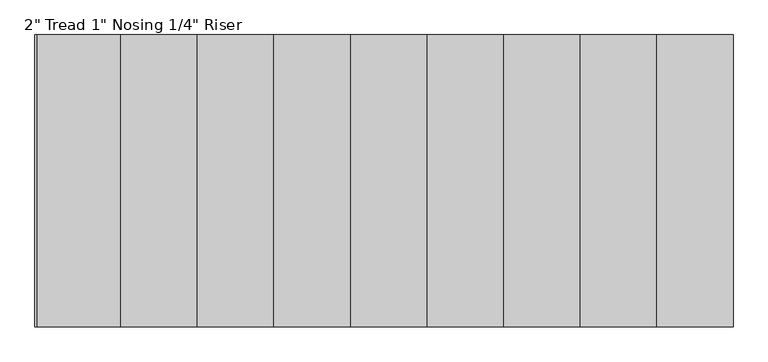
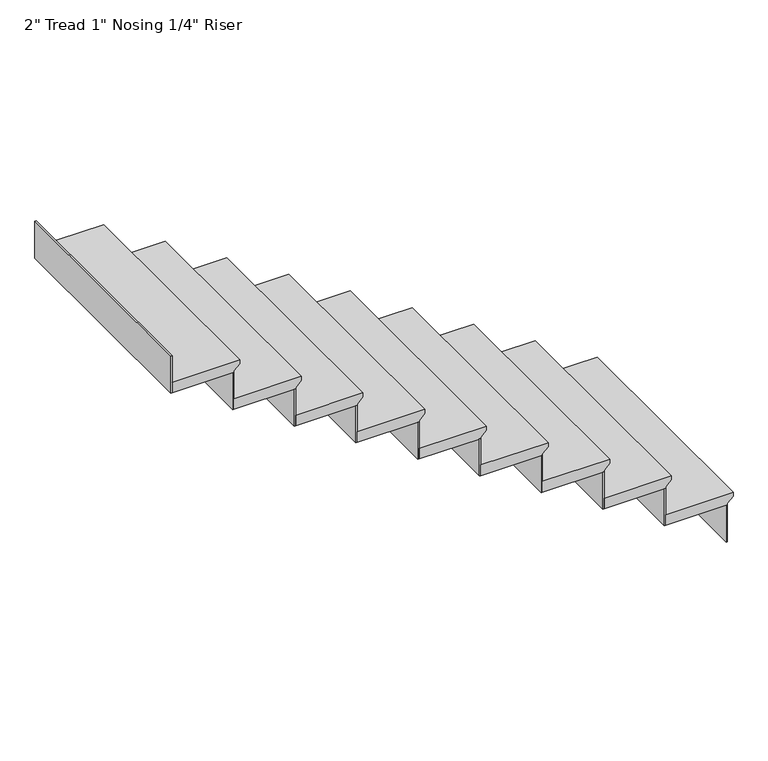
"""IFC4 building model written with IfcOpenShell, lengths in millimetres: stair flight geometry."""

from ifc_helpers import new_model, si_unit, frame, origin, place, context, project, spatial, polyline, outline, extrude, source, transform, mapped, element, save


def stair_flight_a874c81b(model_context):
    return source(origin(), model_context, "Body", "SweptSolid", [
        extrude(outline(polyline([(4959.1783784, 665956.388677), (4959.1783784, 665651.588677), (4908.3783784, 665651.588677), (4908.3783784, 665930.988677), (4914.7283784, 665930.988677), (4940.1283784, 665956.388677), (4959.1783784, 665956.388677)])), frame((0.0, -550482.8413841, 0.0), z_axis=(0.0, 1.0, 0.0), x_axis=(0.0, 0.0, 1.0)), (0.0, 0.0, 1.0), 1066.8),
        extrude(outline(polyline([(665924.638677, -549416.0413841), (665930.988677, -549416.0413841), (665930.988677, -550482.8413841), (665924.638677, -550482.8413841), (665924.638677, -549416.0413841)])), frame((0.0, 0.0, 4731.2648649), z_axis=(0.0, 0.0, 1.0), x_axis=(1.0, 0.0, 0.0)), (0.0, 0.0, 1.0), 177.1135135),
        extrude(outline(polyline([(665645.238677, -549416.0413841), (665651.588677, -549416.0413841), (665651.588677, -550482.8413841), (665645.238677, -550482.8413841), (665645.238677, -549416.0413841)])), frame((0.0, 0.0, 4908.3783784), z_axis=(0.0, 0.0, 1.0), x_axis=(1.0, 0.0, 0.0)), (0.0, 0.0, 1.0), 177.1135135),
        extrude(outline(polyline([(5136.2918919, 665676.988677), (5136.2918919, 665372.188677), (5085.4918919, 665372.188677), (5085.4918919, 665651.588677), (5091.8418919, 665651.588677), (5117.2418919, 665676.988677), (5136.2918919, 665676.988677)])), frame((0.0, -550482.8413841, 0.0), z_axis=(0.0, 1.0, 0.0), x_axis=(0.0, 0.0, 1.0)), (0.0, 0.0, 1.0), 1066.8),
        extrude(outline(polyline([(665365.838677, -549416.0413841), (665372.188677, -549416.0413841), (665372.188677, -550482.8413841), (665365.838677, -550482.8413841), (665365.838677, -549416.0413841)])), frame((0.0, 0.0, 5085.4918919), z_axis=(0.0, 0.0, 1.0), x_axis=(1.0, 0.0, 0.0)), (0.0, 0.0, 1.0), 177.1135135),
        extrude(outline(polyline([(5313.4054054, 665397.588677), (5313.4054054, 665092.788677), (5262.6054054, 665092.788677), (5262.6054054, 665372.188677), (5268.9554054, 665372.188677), (5294.3554054, 665397.588677), (5313.4054054, 665397.588677)])), frame((0.0, -550482.8413841, 0.0), z_axis=(0.0, 1.0, 0.0), x_axis=(0.0, 0.0, 1.0)), (0.0, 0.0, 1.0), 1066.8),
        extrude(outline(polyline([(665086.438677, -549416.0413841), (665092.788677, -549416.0413841), (665092.788677, -550482.8413841), (665086.438677, -550482.8413841), (665086.438677, -549416.0413841)])), frame((0.0, 0.0, 5262.6054054), z_axis=(0.0, 0.0, 1.0), x_axis=(1.0, 0.0, 0.0)), (0.0, 0.0, 1.0), 177.1135135),
        extrude(outline(polyline([(5490.5189189, 665118.188677), (5490.5189189, 664813.388677), (5439.7189189, 664813.388677), (5439.7189189, 665092.788677), (5446.0689189, 665092.788677), (5471.4689189, 665118.188677), (5490.5189189, 665118.188677)])), frame((0.0, -550482.8413841, 0.0), z_axis=(0.0, 1.0, 0.0), x_axis=(0.0, 0.0, 1.0)), (0.0, 0.0, 1.0), 1066.8),
        extrude(outline(polyline([(664807.038677, -549416.0413841), (664813.388677, -549416.0413841), (664813.388677, -550482.8413841), (664807.038677, -550482.8413841), (664807.038677, -549416.0413841)])), frame((0.0, 0.0, 5439.7189189), z_axis=(0.0, 0.0, 1.0), x_axis=(1.0, 0.0, 0.0)), (0.0, 0.0, 1.0), 177.1135135),
        extrude(outline(polyline([(5667.6324324, 664838.788677), (5667.6324324, 664533.988677), (5616.8324324, 664533.988677), (5616.8324324, 664813.388677), (5623.1824324, 664813.388677), (5648.5824324, 664838.788677), (5667.6324324, 664838.788677)])), frame((0.0, -550482.8413841, 0.0), z_axis=(0.0, 1.0, 0.0), x_axis=(0.0, 0.0, 1.0)), (0.0, 0.0, 1.0), 1066.8),
        extrude(outline(polyline([(664527.638677, -549416.0413841), (664533.988677, -549416.0413841), (664533.988677, -550482.8413841), (664527.638677, -550482.8413841), (664527.638677, -549416.0413841)])), frame((0.0, 0.0, 5616.8324324), z_axis=(0.0, 0.0, 1.0), x_axis=(1.0, 0.0, 0.0)), (0.0, 0.0, 1.0), 177.1135135),
        extrude(outline(polyline([(5844.7459459, 664559.388677), (5844.7459459, 664254.588677), (5793.9459459, 664254.588677), (5793.9459459, 664533.988677), (5800.2959459, 664533.988677), (5825.6959459, 664559.388677), (5844.7459459, 664559.388677)])), frame((0.0, -550482.8413841, 0.0), z_axis=(0.0, 1.0, 0.0), x_axis=(0.0, 0.0, 1.0)), (0.0, 0.0, 1.0), 1066.8),
        extrude(outline(polyline([(664248.238677, -549416.0413841), (664254.588677, -549416.0413841), (664254.588677, -550482.8413841), (664248.238677, -550482.8413841), (664248.238677, -549416.0413841)])), frame((0.0, 0.0, 5793.9459459), z_axis=(0.0, 0.0, 1.0), x_axis=(1.0, 0.0, 0.0)), (0.0, 0.0, 1.0), 177.1135135),
        extrude(outline(polyline([(6021.8594595, 664279.988677), (6021.8594595, 663975.188677), (5971.0594595, 663975.188677), (5971.0594595, 664254.588677), (5977.4094595, 664254.588677), (6002.8094595, 664279.988677), (6021.8594595, 664279.988677)])), frame((0.0, -550482.8413841, 0.0), z_axis=(0.0, 1.0, 0.0), x_axis=(0.0, 0.0, 1.0)), (0.0, 0.0, 1.0), 1066.8),
        extrude(outline(polyline([(663968.838677, -549416.0413841), (663975.188677, -549416.0413841), (663975.188677, -550482.8413841), (663968.838677, -550482.8413841), (663968.838677, -549416.0413841)])), frame((0.0, 0.0, 5971.0594595), z_axis=(0.0, 0.0, 1.0), x_axis=(1.0, 0.0, 0.0)), (0.0, 0.0, 1.0), 177.1135135),
        extrude(outline(polyline([(6198.972973, 664000.588677), (6198.972973, 663695.788677), (6148.172973, 663695.788677), (6148.172973, 663975.188677), (6154.522973, 663975.188677), (6179.922973, 664000.588677), (6198.972973, 664000.588677)])), frame((0.0, -550482.8413841, 0.0), z_axis=(0.0, 1.0, 0.0), x_axis=(0.0, 0.0, 1.0)), (0.0, 0.0, 1.0), 1066.8),
        extrude(outline(polyline([(663689.438677, -549416.0413841), (663695.788677, -549416.0413841), (663695.788677, -550482.8413841), (663689.438677, -550482.8413841), (663689.438677, -549416.0413841)])), frame((0.0, 0.0, 6148.172973), z_axis=(0.0, 0.0, 1.0), x_axis=(1.0, 0.0, 0.0)), (0.0, 0.0, 1.0), 177.1135135),
        extrude(outline(polyline([(663410.038677, -549416.0413841), (663416.388677, -549416.0413841), (663416.388677, -550482.8413841), (663410.038677, -550482.8413841), (663410.038677, -549416.0413841)])), frame((0.0, 0.0, 6325.2864865), z_axis=(0.0, 0.0, 1.0), x_axis=(1.0, 0.0, 0.0)), (0.0, 0.0, 1.0), 177.1135135),
        extrude(outline(polyline([(6376.0864865, 663721.188677), (6376.0864865, 663416.388677), (6325.2864865, 663416.388677), (6325.2864865, 663695.788677), (6331.6364865, 663695.788677), (6357.0364865, 663721.188677), (6376.0864865, 663721.188677)])), frame((0.0, -550482.8413841, 0.0), z_axis=(0.0, 1.0, 0.0), x_axis=(0.0, 0.0, 1.0)), (0.0, 0.0, 1.0), 1066.8),
    ])


if __name__ == "__main__":
    model = new_model("IFC4")
    model_context = context("Model", 3, world=origin())
    ifc_project = project(units=[si_unit("LENGTHUNIT", "METRE", prefix="MILLI")], contexts=[model_context])
    site = spatial("IfcSite", under=ifc_project)
    building = spatial("IfcBuilding", under=site)
    placement = place(None, origin())
    stair_flight_shape = stair_flight_a874c81b(model_context)
    element("IfcStairFlight", 1, ObjectType="2\" Tread 1\" Nosing 1/4\" Riser", at=placement, inside=building, context=model_context, shape_type="MappedRepresentation", body=[
        mapped(stair_flight_shape, transform((0.0, 0.0, 0.0), x_axis=(1.0, 0.0, 0.0), y_axis=(0.0, 1.0, 0.0), z_axis=(0.0, 0.0, 1.0))),
    ])
    save(model, "model.ifc")
